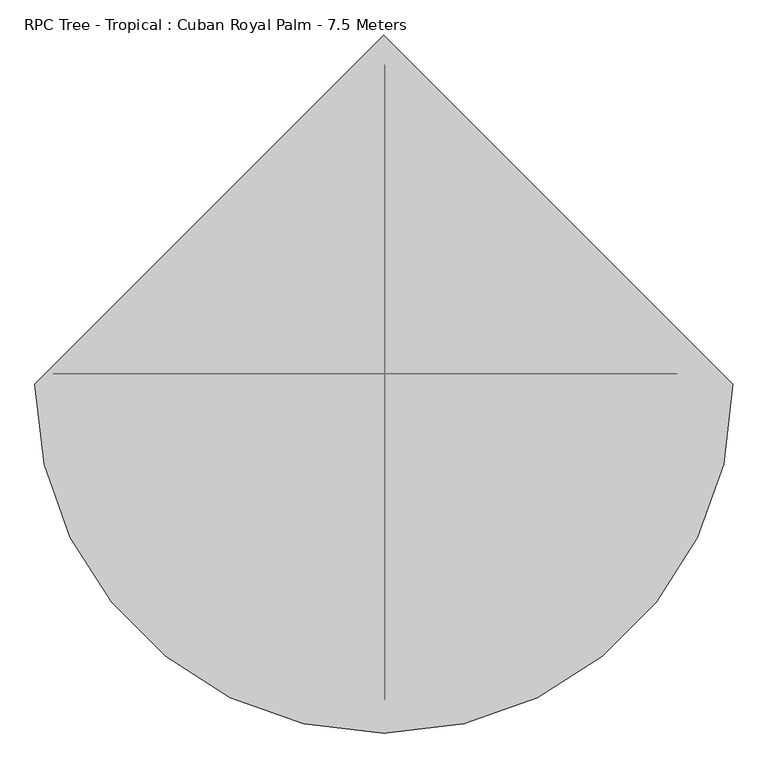
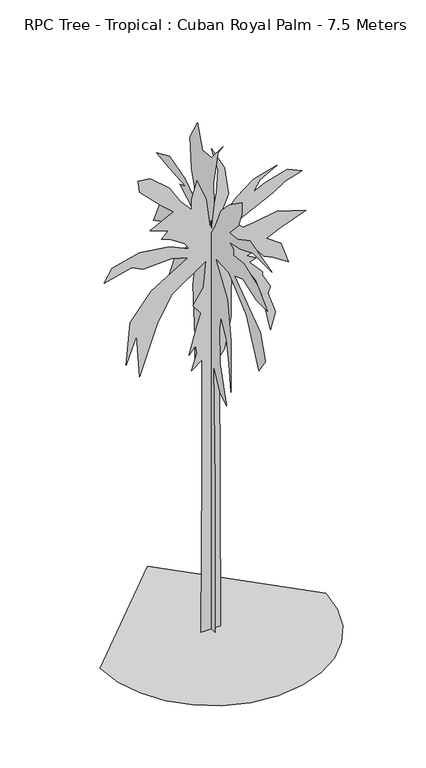
"""IFC4 building model written with IfcOpenShell, lengths in millimetres: geographic element geometry, RPC Tree - Tropical : Cuban Royal Palm - 7.5 Meters."""

import ifcopenshell
import ifcopenshell.guid

model = None  # the IFC model being written
_history = None  # IfcOwnerHistory: only IFC2X3 demands one
_inside = {}  # id of a spatial element -> (the spatial element, [elements in it])
_under = {}  # id of a project, library or spatial element -> (it, [spatial elements below it])
_declared = {}  # id of a project -> (the project, [libraries it declares])
_typed = {}  # id of a type object -> (the type object, [elements of that type])
_made_of = {}  # id of a material, layer set ... -> (it, [elements and type objects made of it])


def new_model(schema):
    """Start an empty IFC model of exactly this schema.

    Asked for "IFC4X3", IfcOpenShell would pick the latest addendum, in which some entities
    have other attributes; the version numbers below select the first issue.
    IFC2X3 requires an IfcOwnerHistory on every rooted entity: one is made here for all.
    """
    global model, _history
    if schema == "IFC4X3":
        model = ifcopenshell.file(schema_version=(4, 3, 0, 0))
    else:
        model = ifcopenshell.file(schema=schema)
    _inside.clear()
    _under.clear()
    _declared.clear()
    _typed.clear()
    _made_of.clear()
    _history = None
    if model.schema == "IFC2X3":
        org = make("IfcOrganization", Name="unknown")
        user = make(
            "IfcPersonAndOrganization",
            ThePerson=make("IfcPerson", FamilyName="unknown"),
            TheOrganization=org,
        )
        app = make(
            "IfcApplication",
            ApplicationDeveloper=org,
            Version="unknown",
            ApplicationFullName="unknown",
            ApplicationIdentifier="unknown",
        )
        _history = make(
            "IfcOwnerHistory",
            OwningUser=user,
            OwningApplication=app,
            ChangeAction="ADDED",
            CreationDate=0,
        )
    return model


def make(cls, **values):
    """One entity of the class cls with the attributes given. An attribute that is None is left unset."""
    return model.create_entity(
        cls, **{name: value for name, value in values.items() if value is not None}
    )


def rooted(cls, **values):
    """An entity with a GlobalId (a new one), such as an element, a storey or a relation."""
    return make(cls, GlobalId=ifcopenshell.guid.new(), OwnerHistory=_history, **values)


def si_unit(unit_type, name, prefix=None):
    """IfcSIUnit, for example si_unit("LENGTHUNIT", "METRE", prefix="MILLI")."""
    return make("IfcSIUnit", UnitType=unit_type, Prefix=prefix, Name=name)


def assignment(units):
    """IfcUnitAssignment: the units of a project."""
    return None if units is None else make("IfcUnitAssignment", Units=units)


def point(xyz):
    """IfcCartesianPoint."""
    return None if xyz is None else make("IfcCartesianPoint", Coordinates=xyz)


def direction(xyz):
    """IfcDirection."""
    return None if xyz is None else make("IfcDirection", DirectionRatios=xyz)


def frame(location, z_axis=None, x_axis=None):
    """IfcAxis2Placement3D, a coordinate frame: its origin and axes. An axis left out is left unset."""
    return make(
        "IfcAxis2Placement3D",
        Location=point(location),
        Axis=direction(z_axis),
        RefDirection=direction(x_axis),
    )


def origin():
    """The frame at (0, 0, 0) with its axes left unset."""
    return frame((0.0, 0.0, 0.0))


def place(relative_to, where):
    """IfcLocalPlacement: puts the frame where relative to a parent placement (None: the world)."""
    return make(
        "IfcLocalPlacement", PlacementRelTo=relative_to, RelativePlacement=where
    )


def context(
    kind, dimensions, precision=None, world=None, true_north=None, identifier=None
):
    """IfcGeometricRepresentationContext, for example the 3D "Model" context."""
    return make(
        "IfcGeometricRepresentationContext",
        ContextIdentifier=identifier,
        ContextType=kind,
        CoordinateSpaceDimension=dimensions,
        Precision=precision,
        WorldCoordinateSystem=world,
        TrueNorth=true_north,
    )


def project(units=None, contexts=None):
    """IfcProject with its units and contexts."""
    return rooted(
        "IfcProject",
        Name="project",
        RepresentationContexts=contexts,
        UnitsInContext=assignment(units),
    )


def spatial(cls, under=None, at=None, **own):
    """A site, building, storey or space (cls), placed at a placement, below another one or the project."""
    s = rooted(cls, ObjectPlacement=at, **own)
    if under is not None:
        _under.setdefault(under.id(), (under, []))[1].append(s)
    return s


def point_list(points):
    """IfcCartesianPointList2D or 3D."""
    cls = (
        "IfcCartesianPointList2D" if len(points[0]) == 2 else "IfcCartesianPointList3D"
    )
    return make(cls, CoordList=points)


def triangles(points, corners, closed=None, point_numbers=None):
    """IfcTriangulatedFaceSet: each triangle names its three corners, points numbered from 1."""
    return make(
        "IfcTriangulatedFaceSet",
        Coordinates=point_list(points),
        Closed=closed,
        CoordIndex=corners,
        PnIndex=point_numbers,
    )


def shape(context_of_items, identifier, shape_type, items):
    """IfcShapeRepresentation: the items that make up one representation, for example the "Body"."""
    return make(
        "IfcShapeRepresentation",
        ContextOfItems=context_of_items,
        RepresentationIdentifier=identifier,
        RepresentationType=shape_type,
        Items=items,
    )


def source(mapping_origin, context_of_items, identifier, shape_type, items):
    """IfcRepresentationMap: a shape defined once, which mapped items show again and again."""
    return make(
        "IfcRepresentationMap",
        MappingOrigin=mapping_origin,
        MappedRepresentation=shape(context_of_items, identifier, shape_type, items),
    )


def transform(
    local_origin,
    x_axis=None,
    y_axis=None,
    z_axis=None,
    scale=None,
    scale2=None,
    scale3=None,
    uniform=True,
):
    """IfcCartesianTransformationOperator3D, or its non-uniform kind. x_axis, y_axis, z_axis: its Axis1, 2, 3."""
    if uniform:
        return make(
            "IfcCartesianTransformationOperator3D",
            Axis1=direction(x_axis),
            Axis2=direction(y_axis),
            LocalOrigin=point(local_origin),
            Scale=scale,
            Axis3=direction(z_axis),
        )
    return make(
        "IfcCartesianTransformationOperator3DnonUniform",
        Axis1=direction(x_axis),
        Axis2=direction(y_axis),
        LocalOrigin=point(local_origin),
        Scale=scale,
        Axis3=direction(z_axis),
        Scale2=scale2,
        Scale3=scale3,
    )


def mapped(mapping_source, mapping_target):
    """IfcMappedItem: shows the shape of a source again, moved by a transform."""
    return make(
        "IfcMappedItem", MappingSource=mapping_source, MappingTarget=mapping_target
    )


def made_of(thing, what):
    """Note that an element or type object is made of a material, layer set ...; save() writes the relation."""
    if what is not None:
        _made_of.setdefault(what.id(), (what, []))[1].append(thing)
    return thing


def element(
    cls,
    number,
    at=None,
    inside=None,
    cuts=None,
    type_object=None,
    material=None,
    context=None,
    identifier="Body",
    shape_type=None,
    held_by="IfcProductDefinitionShape",
    body=None,
    shapes=None,
    **own,
):
    """One element of the class cls, such as IfcWall. Its Tag is "e" and its number.

    at: its placement. inside: the storey or other place that contains it. cuts: it is an
    opening in that element (IfcRelVoidsElement). A single representation is given by context,
    identifier, shape_type and body (its items); several are given by shapes. held_by: the class
    of the entity that holds the representations. save() writes the other relations.
    """
    e = rooted(cls, Tag="e%d" % number, ObjectPlacement=at, **own)
    if body is not None:
        shapes = [shape(context, identifier, shape_type, body)]
    if shapes is not None:
        e.Representation = make(held_by, Representations=shapes)
    if inside is not None:
        _inside.setdefault(inside.id(), (inside, []))[1].append(e)
    if cuts is not None:
        rooted(
            "IfcRelVoidsElement", RelatingBuildingElement=cuts, RelatedOpeningElement=e
        )
    if type_object is not None:
        _typed.setdefault(type_object.id(), (type_object, []))[1].append(e)
    return made_of(e, material)


def aggregate(whole, parts):
    """IfcRelAggregates: a whole, such as a stair, and the parts it consists of."""
    return rooted("IfcRelAggregates", RelatingObject=whole, RelatedObjects=parts)


def save(model, path):
    """Write the relations noted so far, then the file.

    IfcRelAggregates (storeys below a building ...), IfcRelContainedInSpatialStructure (elements
    in a storey), IfcRelDefinesByType, IfcRelAssociatesMaterial and IfcRelDeclares: one each for
    every whole, place, type object, material and project.
    """
    for whole, parts in _under.values():
        aggregate(whole, parts)
    for where, things in _inside.values():
        rooted(
            "IfcRelContainedInSpatialStructure",
            RelatedElements=things,
            RelatingStructure=where,
        )
    for kind, things in _typed.values():
        rooted("IfcRelDefinesByType", RelatedObjects=things, RelatingType=kind)
    for what, things in _made_of.values():
        rooted("IfcRelAssociatesMaterial", RelatedObjects=things, RelatingMaterial=what)
    for by, libraries in _declared.values():
        rooted("IfcRelDeclares", RelatingContext=by, RelatedDefinitions=libraries)
    model.write(path)


def rpc_tree_tropical_cuban_royal_palm_7_5_meters_25244156(model_context):
    return source(origin(), model_context, "Body", "Tessellation", [
        triangles([(-53.329521, -0.0172155, 0.0009289), (-147.4824223, -0.0172239, 0.000933), (-128.6516948, -0.0176557, 2455.3623367), (-128.6514405, -0.0179554, 4131.270797), (-279.295543, -0.0179286, 4018.2957161), (-203.9743774, -0.0179756, 4263.0955994), (-222.8043509, -0.017995, 4376.0703896), (-316.9579788, -0.0179707, 4263.0955994), (-203.974123, -0.0180497, 4677.3703125), (-147.482177, -0.0180825, 4846.8451424), (-260.4655695, -0.0181045, 4997.4949585), (-109.8212127, -0.0181515, 5223.4445389), (-72.1600031, -0.0182238, 5618.8942383), (-561.755246, -0.0181418, 5279.9445786), (-768.8900591, -0.0180688, 4922.1699051), (-1032.519825, -0.017926, 4187.770546), (-1070.1797356, -0.0180388, 4828.0201286), (-1220.8246101, -0.0179615, 4432.5704292), (-1164.3346716, -0.0180751, 5053.9699997), (-863.0449951, -0.0181556, 5430.5946854), (-335.7879704, -0.0182359, 5750.7193314), (-580.5852376, -0.0182387, 5826.0438034), (-976.027343, -0.018218, 5807.1937912), (-1145.5021729, -0.0182241, 5882.5188446), (-1540.9443146, -0.0181899, 5788.3687775), (-1427.9618214, -0.0182286, 5976.6689117), (-1032.519825, -0.0182627, 6070.8439774), (-599.4151929, -0.0182715, 6014.3439377), (-316.9579788, -0.0182603, 5882.5188446), (-373.4504245, -0.0182746, 5976.6689117), (-599.4151929, -0.0182917, 6127.3184372), (-712.4001205, -0.0182935, 6164.9934631), (-618.247728, -0.0183145, 6259.1435303), (-881.8749504, -0.0183198, 6353.2935974), (-542.9252543, -0.0183649, 6522.7681366), (-731.2300758, -0.018387, 6692.2432571), (-1032.519825, -0.0184277, 6993.5428894), (-1051.3497803, -0.0184571, 7163.0174286), (-881.8749504, -0.0184612, 7144.1674164), (-599.4151929, -0.0184298, 6899.3678238), (-448.7703547, -0.0183926, 6654.5682312), (-279.295543, -0.0183663, 6466.2680969), (-279.295543, -0.0183932, 6616.9182037), (-203.974123, -0.0184437, 6880.5428101), (-72.1600031, -0.0183922, 6560.4181641), (-15.6683375, -0.0183139, 6108.4934235), (78.4845898, -0.0184055, 6598.09319), (97.3153263, -0.018467, 6937.0428497), (3.162393, -0.0185268, 7294.8175232), (191.4682185, -0.0184711, 6937.0428497), (247.9601555, -0.0183995, 6522.7681366), (78.4845898, -0.018318, 6108.4934235), (360.9438114, -0.0183876, 6428.6186508), (605.7410422, -0.0184319, 6616.9182037), (944.6906656, -0.0184636, 6711.0682709), (699.8933985, -0.0184293, 6579.2681763), (605.7410422, -0.0183983, 6428.6186508), (775.2158358, -0.0184191, 6503.9431229), (1095.3355402, -0.01845, 6598.09319), (1302.4728241, -0.0184422, 6503.9431229), (1057.6755569, -0.018418, 6428.6186508), (888.2007271, -0.0183904, 6315.6185715), (342.1138198, -0.0183194, 6051.9939651), (455.096204, -0.0183041, 5939.0188843), (605.7410422, -0.0183141, 5957.843898), (944.6906656, -0.018339, 6014.3439377), (1358.9653061, -0.0183335, 5882.5188446), (1001.1831476, -0.0182943, 5750.7193314), (794.0457911, -0.0182684, 5656.5692642), (1001.1831476, -0.0182506, 5505.9191574), (1114.1654955, -0.0181983, 5185.7945114), (888.2007271, -0.0182153, 5336.4446182), (756.3858805, -0.0182197, 5392.9196594), (605.7410422, -0.0182467, 5581.2442108), (605.7410422, -0.0182366, 5524.7441711), (511.5886497, -0.0182258, 5487.0941437), (643.4009892, -0.0182181, 5411.7696716), (549.2486329, -0.0182072, 5374.0946457), (737.5558525, -0.0181784, 5166.9694977), (737.5558525, -0.0181683, 5110.469458), (850.538273, -0.0181362, 4903.3448914), (812.8782898, -0.0181177, 4809.1951149), (925.8607103, -0.0180654, 4489.0704689), (850.538273, -0.0180184, 4244.2705856), (737.5558525, -0.0181111, 4790.3451027), (643.4009892, -0.0181575, 5072.8200119), (473.9261956, -0.0182006, 5355.269632), (304.4513476, -0.0182066, 5430.5946854), (285.6213741, -0.0181385, 5053.9699997), (285.6213741, -0.0180644, 4639.720285), (191.4682185, -0.0179795, 4187.770546), (116.1457994, -0.0179593, 4093.6207695), (134.9762815, -0.0172295, 0.0009206), (0.1930215, 88.1876585, 0.0004872), (0.1930211, 161.0565755, 0.0005002), (0.1930215, 161.0565755, 1798.0106003), (0.1930235, 142.8396006, 4220.8955589), (0.1930219, 215.7080362, 4111.5958351), (0.1930238, 397.879602, 3729.0212219), (0.1930224, 397.879602, 4184.4707474), (0.1930226, 452.5320436, 4949.5949753), (0.1930212, 379.6621093, 5477.8941238), (0.1930204, 525.3994709, 5313.919249), (0.1930227, 780.4416796, 4785.6201004), (0.1930231, 1071.9164028, 4421.295536), (0.193021, 1290.521228, 4075.1707329), (0.1930224, 1035.4814175, 4767.4200485), (0.193022, 871.5265995, 5168.1944229), (0.193022, 507.1819782, 5532.5442764), (0.1930205, 671.1367962, 5496.0941757), (0.1930222, 889.7440922, 5477.8941238), (0.1930219, 1090.1338955, 5514.3192261), (0.1930219, 1436.2610241, 5332.1442993), (0.1930208, 1254.0887135, 5732.9192551), (0.1930227, 1053.6989101, 5732.9192551), (0.1930224, 980.8290121, 6042.618956), (0.1930219, 634.7043543, 5969.7437531), (0.1930206, 416.0970583, 6079.0434769), (0.1930204, 780.4416796, 6279.443454), (0.1930236, 634.7043543, 6334.0936066), (0.1930213, 1035.4814175, 6370.5187088), (0.193023, 1363.3910534, 6406.9682281), (0.1930222, 1035.4814175, 6552.6930542), (0.193022, 652.921847, 6443.3933304), (0.1930203, 343.2271603, 6224.7933014), (0.1930224, 488.9669927, 6698.4428787), (0.1930226, 525.3994709, 7153.8674057), (0.1930219, 343.2271603, 7481.7671585), (0.1930226, 306.794682, 7372.4674347), (0.1930225, 215.7080362, 7135.6423553), (0.1930209, -2.898197, 7153.8674057), (0.1930232, -294.3722026, 7499.9922089), (0.1930217, -166.8530786, 7336.0423325), (0.1930211, -57.5496894, 6807.7431839), (0.193021, -75.7669232, 6498.043483), (0.1930205, 15.3189596, 5987.9688034), (0.1930237, -112.2016361, 6188.343782), (0.1930209, -239.7217594, 6498.043483), (0.1930209, -458.3270388, 6716.6429306), (0.1930205, -768.019182, 6935.2679581), (0.1930205, -768.019182, 6771.2930832), (0.1930212, -676.9343348, 6534.4930023), (0.1930204, -458.3270388, 6297.6685043), (0.1930231, -658.7168421, 6315.8685562), (0.1930203, -968.4089853, 6479.8184326), (0.193022, -1514.9259899, 6334.0936066), (0.1930214, -1041.278956, 6334.0936066), (0.1930223, -731.5867401, 6206.5688324), (0.1930212, -458.3270388, 6151.9186798), (0.1930219, -549.4144295, 6097.2685272), (0.1930215, -549.4144295, 6006.1938538), (0.1930218, -822.67166, 6042.618956), (0.1930224, -1168.7987886, 5915.0941818), (0.193023, -1405.6210339, 5678.2691025), (0.1930208, -1132.3638033, 5678.2691025), (0.1930229, -786.2366747, 5787.5688263), (0.1930214, -585.8493785, 5714.7192032), (0.1930226, -1223.451194, 5241.0696259), (0.1930224, -1350.971172, 4876.720063), (0.1930228, -1187.0162813, 4639.8952744), (0.1930223, -877.3240654, 5295.7197784), (0.1930226, -440.1120532, 5678.2691025), (0.1930235, -112.2016361, 5696.4941528), (0.1930228, -403.6770679, 5241.0696259), (0.1930226, -494.7619878, 4676.3200859), (0.1930204, -494.7619878, 3892.9960968), (0.1930225, -440.1120532, 4293.7704712), (0.1930215, -385.4596115, 4621.670224), (0.1930212, -239.7217594, 4876.720063), (0.1930219, -203.2872827, 4694.5451363), (0.1930229, -221.504521, 4166.245697), (0.1930203, -385.4596115, 3619.7212074), (0.1930216, -221.504521, 3729.0212219), (0.1930209, -57.5496894, 4038.7209229), (0.1930231, -93.9844068, 2253.4402142), (0.1930206, -93.9844068, 0.0004546), (-1626.8666862, -48.3554514, 0.0005339), (-1583.9691593, -420.1520797, 0.0004655), (-1461.7992908, -761.5891966, 0.0003991), (-1270.1394779, -1062.8838873, 0.0003369), (-1018.7723356, -1314.2511749, 0.0002809), (-717.4776449, -1505.9109879, 0.0002335), (-376.0429261, -1628.0808563, 0.0001967), (-4.2444493, -1670.9782379, 0.0001728), (367.5538004, -1628.0808563, 0.0001642), (708.9884102, -1505.9109879, 0.0001711), (1010.2831009, -1314.2511749, 0.0001922), (1261.6503159, -1062.8838873, 0.0002262), (1453.3101288, -761.5891966, 0.0002717), (1575.4799973, -420.1520797, 0.0003274), (1618.3775242, -48.3554514, 0.000392), (-4.2447494, 1574.2658272, 0.000298)], [[54, 55, 56], [48, 49, 50], [17, 18, 19], [15, 16, 17], [7, 8, 9], [83, 84, 85], [82, 83, 85], [4, 5, 6], [70, 71, 72], [66, 67, 68], [43, 44, 45], [59, 60, 61], [24, 25, 26], [24, 26, 27], [33, 34, 35], [76, 77, 78], [58, 59, 61], [58, 61, 62], [31, 32, 33], [42, 43, 45], [42, 45, 46], [37, 38, 39], [54, 56, 57], [53, 54, 57], [23, 24, 27], [23, 27, 28], [22, 23, 28], [22, 28, 29], [21, 22, 29], [58, 62, 63], [57, 58, 63], [53, 57, 63], [52, 53, 63], [36, 37, 39], [36, 39, 40], [36, 40, 41], [35, 36, 41], [35, 41, 42], [69, 70, 72], [69, 72, 73], [69, 73, 74], [65, 66, 68], [65, 68, 69], [65, 69, 74], [64, 65, 74], [47, 48, 50], [47, 50, 51], [46, 47, 51], [46, 51, 52], [33, 35, 42], [82, 85, 86], [81, 82, 86], [80, 81, 86], [33, 42, 46], [31, 33, 46], [30, 31, 46], [29, 30, 46], [15, 17, 19], [15, 19, 20], [14, 15, 20], [14, 20, 21], [13, 14, 21], [92, 93, 1], [92, 1, 2], [92, 2, 3], [92, 3, 4], [80, 86, 87], [79, 80, 87], [78, 79, 87], [76, 78, 87], [76, 87, 88], [13, 21, 29], [13, 29, 46], [13, 46, 52], [13, 52, 63], [13, 63, 64], [13, 64, 74], [13, 74, 75], [13, 75, 76], [13, 76, 88], [12, 13, 88], [12, 88, 89], [11, 12, 89], [10, 11, 89], [10, 89, 90], [9, 10, 90], [9, 90, 91], [7, 9, 91], [6, 7, 91], [4, 6, 91], [92, 4, 91], [131, 132, 133], [165, 166, 167], [105, 106, 107], [145, 146, 147], [165, 167, 168], [98, 99, 100], [131, 133, 134], [121, 122, 123], [104, 105, 107], [112, 113, 114], [171, 172, 173], [171, 173, 174], [153, 154, 155], [127, 128, 129], [118, 119, 120], [112, 114, 115], [139, 140, 141], [139, 141, 142], [159, 160, 161], [158, 159, 161], [157, 158, 161], [157, 161, 162], [104, 107, 108], [103, 104, 108], [103, 108, 109], [102, 103, 109], [127, 129, 130], [121, 123, 124], [120, 121, 124], [120, 124, 125], [118, 120, 125], [153, 155, 156], [152, 153, 156], [151, 152, 156], [151, 156, 157], [126, 127, 130], [145, 147, 148], [144, 145, 148], [144, 148, 149], [143, 144, 149], [139, 142, 143], [138, 139, 143], [137, 138, 143], [137, 143, 149], [175, 176, 94], [175, 94, 95], [175, 95, 96], [175, 96, 97], [174, 175, 97], [111, 112, 115], [115, 116, 117], [111, 115, 117], [110, 111, 117], [109, 110, 117], [165, 168, 169], [164, 165, 169], [130, 131, 134], [126, 130, 134], [126, 134, 135], [125, 126, 135], [125, 135, 136], [118, 125, 136], [151, 157, 162], [171, 174, 97], [170, 171, 97], [109, 117, 118], [109, 118, 136], [102, 109, 136], [97, 98, 100], [97, 100, 101], [170, 97, 101], [169, 170, 101], [169, 101, 102], [164, 169, 102], [163, 164, 102], [163, 102, 136], [151, 162, 163], [151, 163, 136], [151, 136, 137], [151, 137, 149], [151, 149, 150], [191, 192, 177], [190, 191, 177], [190, 177, 178], [189, 190, 178], [189, 178, 179], [189, 179, 180], [188, 189, 180], [187, 188, 180], [187, 180, 181], [187, 181, 182], [187, 182, 183], [187, 183, 184], [187, 184, 185], [187, 185, 186]], closed=False),
    ])


if __name__ == "__main__":
    model = new_model("IFC4")
    model_context = context("Model", 3, world=origin())
    ifc_project = project(units=[si_unit("LENGTHUNIT", "METRE", prefix="MILLI")], contexts=[model_context])
    site = spatial("IfcSite", under=ifc_project)
    building = spatial("IfcBuilding", under=site)
    placement = place(None, origin())
    rpc_tree_tropical_cuban_royal_palm_7_5_meters_shape = rpc_tree_tropical_cuban_royal_palm_7_5_meters_25244156(model_context)
    element("IfcGeographicElement", 1, ObjectType="RPC Tree - Tropical : Cuban Royal Palm - 7.5 Meters", at=placement, inside=building, context=model_context, shape_type="MappedRepresentation", body=[
        mapped(rpc_tree_tropical_cuban_royal_palm_7_5_meters_shape, transform((0.0, 0.0, 0.0), x_axis=(1.0, 0.0, 0.0), y_axis=(0.0, 1.0, 0.0), z_axis=(0.0, 0.0, 1.0))),
    ])
    save(model, "model.ifc")

# Revit data of these elements
# Type "RPC Tree - Tropical : Cuban Royal Palm - 7.5 Meters"
#   built-in parameter 1005198 = "{2, 15},{39, RPC-16-FVGV-NKG0-7NHH-C000-ST1L-LVER-AU},{1, 0},{1, 0},{2, 13},{1, 8},{5, Color},{1, 0},{1, 0},{3, 0.8},{3, 0.8},{3, 0.8},{1, 8},{7, BBoxMin},{1, 0},{1, 0},{1, 0},{1, 0},{1, 0},{1, 8},{7, BBoxMax},{1, 0},{1, 0},{1, 0},{1, 0},{1, 0},{2, 11},{9, RPCTypeId},{1, 0},{1, 0},{39, RPC-16-FVGV-NKG0-7NHH-C000-ST1L-LVER-AU},{1, 6},{14, RPCPlantHeight},{1, 0},{1, 0},{7, 24.6063},{2, 11},{7, keyword},{1, 0},{1, 0},{35, :RPCs:Trees [Tropical]:Geometry:RPC},{2, 11},{8, category},{1, 0},{1, 0},{16, Trees [Tropical]},{2, 11},{12, LocalizedUID},{1, 0},{1, 0},{16, Cuban Royal Palm},{2, 14},{6, Height},{1, 0},{1, 0},{7, 24.6063},{1, 2},{16, Cast Reflections},{1, 0},{1, 0},{1, 0},{1, 2},{12, Cast Shadows},{1, 0},{1, 0},{1, 1},{1, 2},{9, Lock View},{1, 0},{1, 0},{1, 0},{1, 4},{5, ViewC},{1, 0},{1, 0},{1, 0},{21, assetlibrary_base.fbx},{1, 5},"
#   built-in parameter 1005195 = "RPC-16-FVGV-NKG0-7NHH-C000-ST1L-LVER-AU"
#   Type Comments = "Cuban Royal Palm"
#   Height = 7500 mm
#   Plan Symbol = element 242927
#   Description = (empty or 0)
